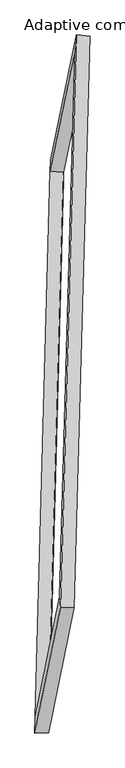
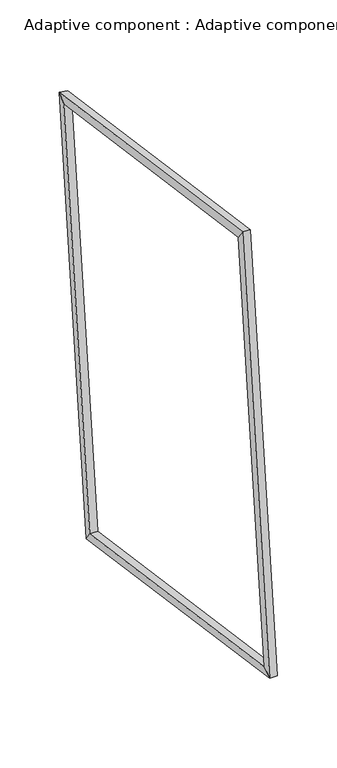
"""IFC4 building model written with IfcOpenShell, lengths in millimetres: proxy geometry, Adaptive component : Adaptive component."""

from ifc_helpers import new_model, si_unit, origin, place, context, project, spatial, faceted_brep, source, transform, mapped, element, save


def adaptive_component_adaptive_component_bd8922ac(model_context):
    return source(origin(), model_context, "Body", "Brep", [
        faceted_brep([(71.5639696, 1164.9188089, 2782.6356426), (136.2124461, 1158.9957453, 2778.0224347), (64.5685226, -1430.3262839, 3226.6733245), (-0.2589925, -1430.8739532, 3232.4077139), (78.8877634, 1239.7662671, 2835.3938664), (3.5264844, -1483.9067297, 3307.3236996), (143.5362398, 1233.8432035, 2830.7806585), (68.3539995, -1483.3590603, 3301.5893102), (-53.3208463, -2001.6081903, -89.2208727), (-118.3783965, -2003.2705902, -89.9567188), (-119.1390722, -2078.3336377, -142.9111369), (-54.0815221, -2076.6712378, -142.1752908), (18.3230771, 587.7138389, -537.8717625), (-46.5554344, 592.522172, -539.7287902), (-43.7777933, 645.3393591, -614.8409702), (21.1007182, 640.531026, -612.9839425)], [[[0, 1, 2, 3]], [[4, 0, 3, 5]], [[6, 4, 5, 7]], [[1, 6, 7, 2]], [[3, 2, 8, 9]], [[5, 3, 9, 10]], [[7, 5, 10, 11]], [[2, 7, 11, 8]], [[9, 8, 12, 13]], [[10, 9, 13, 14]], [[11, 10, 14, 15]], [[8, 11, 15, 12]], [[13, 12, 1, 0]], [[14, 13, 0, 4]], [[15, 14, 4, 6]], [[12, 15, 6, 1]]]),
    ])


if __name__ == "__main__":
    model = new_model("IFC4")
    model_context = context("Model", 3, world=origin())
    ifc_project = project(units=[si_unit("LENGTHUNIT", "METRE", prefix="MILLI")], contexts=[model_context])
    site = spatial("IfcSite", under=ifc_project)
    building = spatial("IfcBuilding", under=site)
    placement = place(None, origin())
    adaptive_component_adaptive_component_shape = adaptive_component_adaptive_component_bd8922ac(model_context)
    element("IfcBuildingElementProxy", 1, Name="Adaptive component : Adaptive component", ObjectType="Adaptive component : Adaptive component", at=placement, inside=building, context=model_context, shape_type="MappedRepresentation", body=[
        mapped(adaptive_component_adaptive_component_shape, transform((0.0, 0.0, 0.0), x_axis=(1.0, 0.0, 0.0), y_axis=(0.0, 1.0, 0.0), z_axis=(0.0, 0.0, 1.0))),
    ])
    save(model, "model.ifc")

# Revit data of these elements
# Type "Adaptive component : Adaptive component"
#   r [instance default] = 2063.125 mm
#   2r [instance default] = 4126.251 mm
#   Number [instance default] = 5
#   Default Elevation = 0
# Element 1 (IfcBuildingElementProxy, "Adaptive component : Adaptive component")
#   r = 2229.295 mm
#   2r = 4458.59 mm
#   Number = 11
